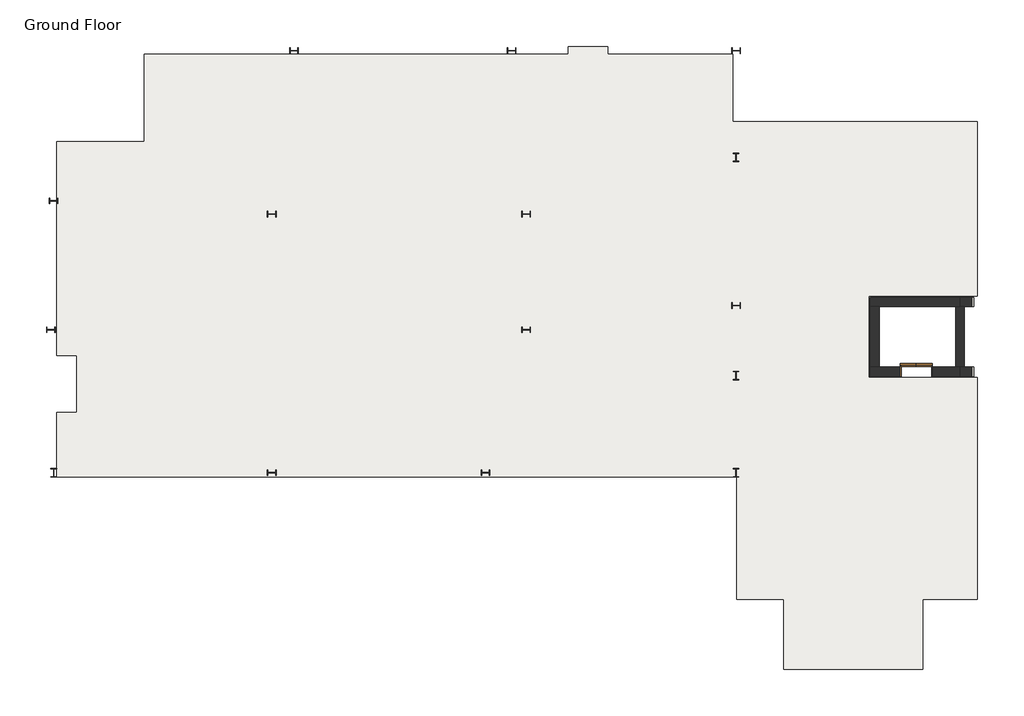
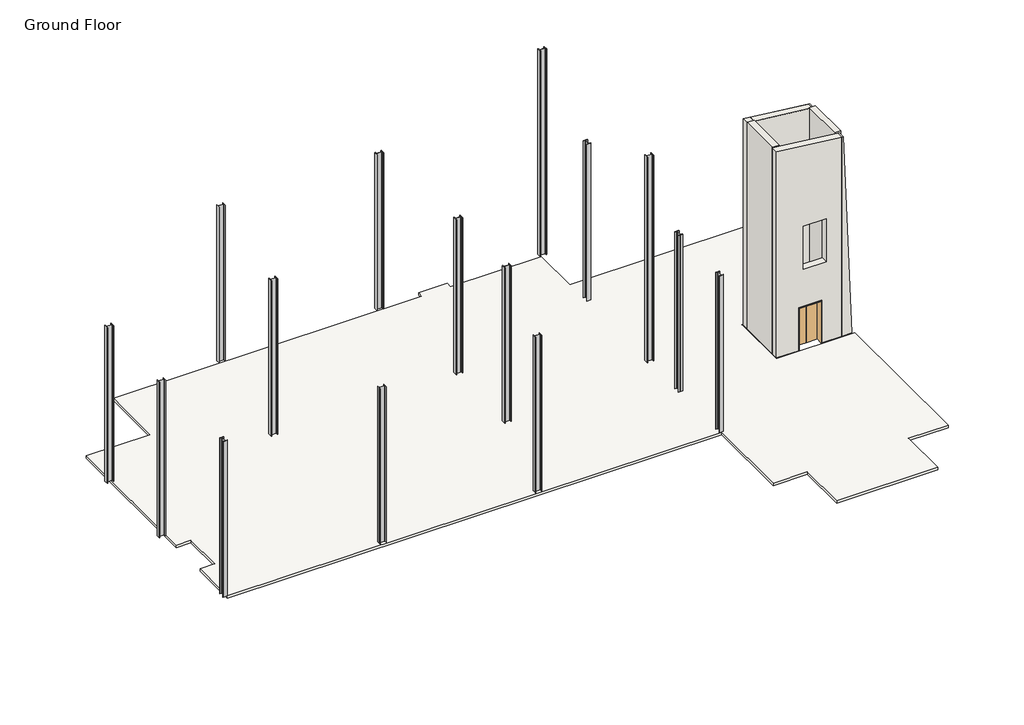
# One storey: 15 columns, 7 walls, 1 door, 1 slab.
"""IFC4 building model written with IfcOpenShell, lengths in millimetres."""

import ifcopenshell
import ifcopenshell.guid

model = None  # the IFC model being written
_history = None  # IfcOwnerHistory: only IFC2X3 demands one
_inside = {}  # id of a spatial element -> (the spatial element, [elements in it])
_under = {}  # id of a project, library or spatial element -> (it, [spatial elements below it])
_declared = {}  # id of a project -> (the project, [libraries it declares])
_typed = {}  # id of a type object -> (the type object, [elements of that type])
_made_of = {}  # id of a material, layer set ... -> (it, [elements and type objects made of it])


def new_model(schema):
    """Start an empty IFC model of exactly this schema.

    Asked for "IFC4X3", IfcOpenShell would pick the latest addendum, in which some entities
    have other attributes; the version numbers below select the first issue.
    IFC2X3 requires an IfcOwnerHistory on every rooted entity: one is made here for all.
    """
    global model, _history
    if schema == "IFC4X3":
        model = ifcopenshell.file(schema_version=(4, 3, 0, 0))
    else:
        model = ifcopenshell.file(schema=schema)
    _inside.clear()
    _under.clear()
    _declared.clear()
    _typed.clear()
    _made_of.clear()
    _history = None
    if model.schema == "IFC2X3":
        org = make("IfcOrganization", Name="unknown")
        user = make(
            "IfcPersonAndOrganization",
            ThePerson=make("IfcPerson", FamilyName="unknown"),
            TheOrganization=org,
        )
        app = make(
            "IfcApplication",
            ApplicationDeveloper=org,
            Version="unknown",
            ApplicationFullName="unknown",
            ApplicationIdentifier="unknown",
        )
        _history = make(
            "IfcOwnerHistory",
            OwningUser=user,
            OwningApplication=app,
            ChangeAction="ADDED",
            CreationDate=0,
        )
    return model


def make(cls, **values):
    """One entity of the class cls with the attributes given. An attribute that is None is left unset."""
    return model.create_entity(
        cls, **{name: value for name, value in values.items() if value is not None}
    )


def rooted(cls, **values):
    """An entity with a GlobalId (a new one), such as an element, a storey or a relation."""
    return make(cls, GlobalId=ifcopenshell.guid.new(), OwnerHistory=_history, **values)


def si_unit(unit_type, name, prefix=None):
    """IfcSIUnit, for example si_unit("LENGTHUNIT", "METRE", prefix="MILLI")."""
    return make("IfcSIUnit", UnitType=unit_type, Prefix=prefix, Name=name)


def assignment(units):
    """IfcUnitAssignment: the units of a project."""
    return None if units is None else make("IfcUnitAssignment", Units=units)


def point(xyz):
    """IfcCartesianPoint."""
    return None if xyz is None else make("IfcCartesianPoint", Coordinates=xyz)


def direction(xyz):
    """IfcDirection."""
    return None if xyz is None else make("IfcDirection", DirectionRatios=xyz)


def frame(location, z_axis=None, x_axis=None):
    """IfcAxis2Placement3D, a coordinate frame: its origin and axes. An axis left out is left unset."""
    return make(
        "IfcAxis2Placement3D",
        Location=point(location),
        Axis=direction(z_axis),
        RefDirection=direction(x_axis),
    )


def frame_2d(location, x_axis=None):
    """IfcAxis2Placement2D, a coordinate frame in the plane: its origin and x axis."""
    return make(
        "IfcAxis2Placement2D", Location=point(location), RefDirection=direction(x_axis)
    )


def origin():
    """The frame at (0, 0, 0) with its axes left unset."""
    return frame((0.0, 0.0, 0.0))


def origin_with_axes():
    """The frame at (0, 0, 0) with the z axis (0, 0, 1) and the x axis (1, 0, 0) written out."""
    return frame((0.0, 0.0, 0.0), z_axis=(0.0, 0.0, 1.0), x_axis=(1.0, 0.0, 0.0))


def place(relative_to, where):
    """IfcLocalPlacement: puts the frame where relative to a parent placement (None: the world)."""
    return make(
        "IfcLocalPlacement", PlacementRelTo=relative_to, RelativePlacement=where
    )


def context(
    kind, dimensions, precision=None, world=None, true_north=None, identifier=None
):
    """IfcGeometricRepresentationContext, for example the 3D "Model" context."""
    return make(
        "IfcGeometricRepresentationContext",
        ContextIdentifier=identifier,
        ContextType=kind,
        CoordinateSpaceDimension=dimensions,
        Precision=precision,
        WorldCoordinateSystem=world,
        TrueNorth=true_north,
    )


def project(units=None, contexts=None):
    """IfcProject with its units and contexts."""
    return rooted(
        "IfcProject",
        Name="project",
        RepresentationContexts=contexts,
        UnitsInContext=assignment(units),
    )


def spatial(cls, under=None, at=None, **own):
    """A site, building, storey or space (cls), placed at a placement, below another one or the project."""
    s = rooted(cls, ObjectPlacement=at, **own)
    if under is not None:
        _under.setdefault(under.id(), (under, []))[1].append(s)
    return s


def polyline(points):
    """IfcPolyline through the points."""
    return make("IfcPolyline", Points=[point(p) for p in points])


def circle_curve(where, radius):
    """IfcCircle in the frame where."""
    return make("IfcCircle", Position=where, Radius=radius)


def trimmed(basis, trim1, trim2, sense, master):
    """IfcTrimmedCurve: the piece of a basis curve between two trims."""
    return make(
        "IfcTrimmedCurve",
        BasisCurve=basis,
        Trim1=trim1,
        Trim2=trim2,
        SenseAgreement=sense,
        MasterRepresentation=master,
    )


def segment(curve, same_sense, transition):
    """IfcCompositeCurveSegment."""
    return make(
        "IfcCompositeCurveSegment",
        Transition=transition,
        SameSense=same_sense,
        ParentCurve=curve,
    )


def composite_curve(segments, self_intersect=None):
    """IfcCompositeCurve: segments joined end to end."""
    return make("IfcCompositeCurve", Segments=segments, SelfIntersect=self_intersect)


def outline(outer, holes=None, kind="AREA"):
    """IfcArbitraryClosedProfileDef: a profile drawn as a closed curve; with holes, ...WithVoids."""
    if holes is None:
        return make("IfcArbitraryClosedProfileDef", ProfileType=kind, OuterCurve=outer)
    return make(
        "IfcArbitraryProfileDefWithVoids",
        ProfileType=kind,
        OuterCurve=outer,
        InnerCurves=holes,
    )


def extrude(swept, where, along, depth):
    """IfcExtrudedAreaSolid: the profile swept, set in the frame where, extruded along a direction by depth."""
    return make(
        "IfcExtrudedAreaSolid",
        SweptArea=swept,
        Position=where,
        ExtrudedDirection=direction(along),
        Depth=depth,
    )


def faces_of(points, faces, orient=None, outer=None):
    """IfcFace entities. A face is a list of loops; a loop is a list of indices into points, from 0.

    orient and outer hold one flag for each loop. By default every Orientation is true, the
    first loop of a face is its IfcFaceOuterBound and the others are IfcFaceBound.
    """
    made = []
    for i, loops in enumerate(faces):
        bounds = []
        for j, loop in enumerate(loops):
            is_outer = j == 0 if outer is None else outer[i][j]
            bounds.append(
                make(
                    "IfcFaceOuterBound" if is_outer else "IfcFaceBound",
                    Bound=make("IfcPolyLoop", Polygon=[points[k] for k in loop]),
                    Orientation=True if orient is None else orient[i][j],
                )
            )
        made.append(make("IfcFace", Bounds=bounds))
    return made


def faceted_brep(points, faces, orient=None, outer=None, voids=None):
    """IfcFacetedBrep: a solid bounded by flat faces; with voids (closed shells), ...WithVoids."""
    shared = [point(p) for p in points]
    hull = make("IfcClosedShell", CfsFaces=faces_of(shared, faces, orient, outer))
    if voids is None:
        return make("IfcFacetedBrep", Outer=hull)
    return make(
        "IfcFacetedBrepWithVoids",
        Outer=hull,
        Voids=[
            make(cls, CfsFaces=faces_of(shared, fs, o, b)) for cls, fs, o, b in voids
        ],
    )


def shape(context_of_items, identifier, shape_type, items):
    """IfcShapeRepresentation: the items that make up one representation, for example the "Body"."""
    return make(
        "IfcShapeRepresentation",
        ContextOfItems=context_of_items,
        RepresentationIdentifier=identifier,
        RepresentationType=shape_type,
        Items=items,
    )


def source(mapping_origin, context_of_items, identifier, shape_type, items):
    """IfcRepresentationMap: a shape defined once, which mapped items show again and again."""
    return make(
        "IfcRepresentationMap",
        MappingOrigin=mapping_origin,
        MappedRepresentation=shape(context_of_items, identifier, shape_type, items),
    )


def transform(
    local_origin,
    x_axis=None,
    y_axis=None,
    z_axis=None,
    scale=None,
    scale2=None,
    scale3=None,
    uniform=True,
):
    """IfcCartesianTransformationOperator3D, or its non-uniform kind. x_axis, y_axis, z_axis: its Axis1, 2, 3."""
    if uniform:
        return make(
            "IfcCartesianTransformationOperator3D",
            Axis1=direction(x_axis),
            Axis2=direction(y_axis),
            LocalOrigin=point(local_origin),
            Scale=scale,
            Axis3=direction(z_axis),
        )
    return make(
        "IfcCartesianTransformationOperator3DnonUniform",
        Axis1=direction(x_axis),
        Axis2=direction(y_axis),
        LocalOrigin=point(local_origin),
        Scale=scale,
        Axis3=direction(z_axis),
        Scale2=scale2,
        Scale3=scale3,
    )


def mapped(mapping_source, mapping_target):
    """IfcMappedItem: shows the shape of a source again, moved by a transform."""
    return make(
        "IfcMappedItem", MappingSource=mapping_source, MappingTarget=mapping_target
    )


def made_of(thing, what):
    """Note that an element or type object is made of a material, layer set ...; save() writes the relation."""
    if what is not None:
        _made_of.setdefault(what.id(), (what, []))[1].append(thing)
    return thing


def element(
    cls,
    number,
    at=None,
    inside=None,
    cuts=None,
    type_object=None,
    material=None,
    context=None,
    identifier="Body",
    shape_type=None,
    held_by="IfcProductDefinitionShape",
    body=None,
    shapes=None,
    **own,
):
    """One element of the class cls, such as IfcWall. Its Tag is "e" and its number.

    at: its placement. inside: the storey or other place that contains it. cuts: it is an
    opening in that element (IfcRelVoidsElement). A single representation is given by context,
    identifier, shape_type and body (its items); several are given by shapes. held_by: the class
    of the entity that holds the representations. save() writes the other relations.
    """
    e = rooted(cls, Tag="e%d" % number, ObjectPlacement=at, **own)
    if body is not None:
        shapes = [shape(context, identifier, shape_type, body)]
    if shapes is not None:
        e.Representation = make(held_by, Representations=shapes)
    if inside is not None:
        _inside.setdefault(inside.id(), (inside, []))[1].append(e)
    if cuts is not None:
        rooted(
            "IfcRelVoidsElement", RelatingBuildingElement=cuts, RelatedOpeningElement=e
        )
    if type_object is not None:
        _typed.setdefault(type_object.id(), (type_object, []))[1].append(e)
    return made_of(e, material)


def aggregate(whole, parts):
    """IfcRelAggregates: a whole, such as a stair, and the parts it consists of."""
    return rooted("IfcRelAggregates", RelatingObject=whole, RelatedObjects=parts)


def save(model, path):
    """Write the relations noted so far, then the file.

    IfcRelAggregates (storeys below a building ...), IfcRelContainedInSpatialStructure (elements
    in a storey), IfcRelDefinesByType, IfcRelAssociatesMaterial and IfcRelDeclares: one each for
    every whole, place, type object, material and project.
    """
    for whole, parts in _under.values():
        aggregate(whole, parts)
    for where, things in _inside.values():
        rooted(
            "IfcRelContainedInSpatialStructure",
            RelatedElements=things,
            RelatingStructure=where,
        )
    for kind, things in _typed.values():
        rooted("IfcRelDefinesByType", RelatedObjects=things, RelatingType=kind)
    for what, things in _made_of.values():
        rooted("IfcRelAssociatesMaterial", RelatedObjects=things, RelatingMaterial=what)
    for by, libraries in _declared.values():
        rooted("IfcRelDeclares", RelatingContext=by, RelatedDefinitions=libraries)
    model.write(path)


def w_wide_flange_column_w12x40_bfea6e2c(model_context):
    return source(origin(), model_context, "Body", "SweptSolid", [
        extrude(outline(composite_curve([segment(polyline([(101.6496094, 151.6558594), (101.6496094, 138.5589844), (25.5984375, 138.5589844)]), True, "CONTINUOUS"), segment(trimmed(circle_curve(frame_2d((25.5984375, 116.7308594)), 21.828125), [point((25.5984375, 138.5589844))], [point((3.7703125, 116.7308594))], True, "CARTESIAN"), True, "CONTINUOUS"), segment(polyline([(3.7703125, 116.7308594), (3.7703125, -116.7308594)]), True, "CONTINUOUS"), segment(trimmed(circle_curve(frame_2d((25.5984375, -116.7308594)), 21.828125), [point((3.7703125, -116.7308594))], [point((25.5984375, -138.5589844))], True, "CARTESIAN"), True, "CONTINUOUS"), segment(polyline([(25.5984375, -138.5589844), (101.6496094, -138.5589844), (101.6496094, -151.6558594), (-101.6496094, -151.6558594), (-101.6496094, -138.5589844), (-25.5984375, -138.5589844)]), True, "CONTINUOUS"), segment(trimmed(circle_curve(frame_2d((-25.5984375, -116.7308594)), 21.828125), [point((-25.5984375, -138.5589844))], [point((-3.7703125, -116.7308594))], True, "CARTESIAN"), True, "CONTINUOUS"), segment(polyline([(-3.7703125, -116.7308594), (-3.7703125, 116.7308594)]), True, "CONTINUOUS"), segment(trimmed(circle_curve(frame_2d((-25.5984375, 116.7308594)), 21.828125), [point((-3.7703125, 116.7308594))], [point((-25.5984375, 138.5589844))], True, "CARTESIAN"), True, "CONTINUOUS"), segment(polyline([(-25.5984375, 138.5589844), (-101.6496094, 138.5589844), (-101.6496094, 151.6558594), (101.6496094, 151.6558594)]), True, "CONTINUOUS")], self_intersect=False)), frame((0.0, 0.0, 30480.0), z_axis=(0.0, 0.0, 1.0), x_axis=(1.0, 0.0, 0.0)), (0.0, 0.0, 1.0), 7924.8),
    ])


def door_aaeb5b8c(model_context):
    return source(origin(), model_context, "Body", "SweptSolid", [
        extrude(outline(polyline([(0.0, 234.95), (0.0, 279.4), (558.8, 279.4), (558.8, 234.95), (0.0, 234.95)])), origin_with_axes(), (0.0, 0.0, 1.0), 2184.4),
        extrude(outline(polyline([(0.0, 234.95), (-558.8, 234.95), (-558.8, 279.4), (0.0, 279.4), (0.0, 234.95)])), origin_with_axes(), (0.0, 0.0, 1.0), 2184.4),
        extrude(outline(polyline([(-533.4, -165.1), (-558.8, -165.1), (-558.8, 177.8), (-533.4, 177.8), (-533.4, -165.1)])), origin_with_axes(), (0.0, 0.0, 1.0), 2184.4),
        extrude(outline(polyline([(558.8, -165.1), (533.4, -165.1), (533.4, 177.8), (558.8, 177.8), (558.8, -165.1)])), origin_with_axes(), (0.0, 0.0, 1.0), 2184.4),
        extrude(outline(polyline([(482.6, 165.1), (482.6, -165.1), (-482.6, -165.1), (-482.6, 165.1), (482.6, 165.1)])), frame((0.0, 0.0, 2133.6), z_axis=(0.0, 0.0, 1.0), x_axis=(1.0, 0.0, 0.0)), (0.0, 0.0, 1.0), 50.8),
        extrude(outline(polyline([(0.0, 177.8), (0.0, 222.25), (558.8, 222.25), (558.8, 177.8), (0.0, 177.8)])), origin_with_axes(), (0.0, 0.0, 1.0), 2184.4),
        extrude(outline(polyline([(0.0, 177.8), (-558.8, 177.8), (-558.8, 222.25), (0.0, 222.25), (0.0, 177.8)])), origin_with_axes(), (0.0, 0.0, 1.0), 2184.4),
    ])


model = new_model("IFC4")

# Units and contexts
model_context = context("Model", 3, world=origin())
ifc_project = project(units=[si_unit("LENGTHUNIT", "METRE", prefix="MILLI")], contexts=[model_context])

# Site, building, storey
site = spatial("IfcSite", under=ifc_project)
building = spatial("IfcBuilding", under=site)
storey = spatial("IfcBuildingStorey", under=building, Name="Ground Floor", Elevation=30480.0)

# Columns
placement = place(None, origin())
element("IfcColumn", 1, ObjectType="W-Wide Flange-Column : W12X40", at=placement, inside=storey, context=model_context, shape_type="SweptSolid", body=[
    extrude(outline(composite_curve([segment(polyline([(13669.3791487, -6791.0746401), (13669.3791487, -6804.1715151), (13593.3279768, -6804.1715151)]), True, "CONTINUOUS"), segment(trimmed(circle_curve(frame_2d((13593.3279768, -6825.9996401)), 21.828125), [point((13593.3279768, -6804.1715151))], [point((13571.4998518, -6825.9996401))], True, "CARTESIAN"), True, "CONTINUOUS"), segment(polyline([(13571.4998518, -6825.9996401), (13571.4998518, -7059.4613589)]), True, "CONTINUOUS"), segment(trimmed(circle_curve(frame_2d((13593.3279768, -7059.4613589)), 21.828125), [point((13571.4998518, -7059.4613589))], [point((13593.3279768, -7081.2894839))], True, "CARTESIAN"), True, "CONTINUOUS"), segment(polyline([(13593.3279768, -7081.2894839), (13669.3791487, -7081.2894839), (13669.3791487, -7094.3863589), (13466.0799299, -7094.3863589), (13466.0799299, -7081.2894839), (13542.1311018, -7081.2894839)]), True, "CONTINUOUS"), segment(trimmed(circle_curve(frame_2d((13542.1311018, -7059.4613589)), 21.828125), [point((13542.1311018, -7081.2894839))], [point((13563.9592268, -7059.4613589))], True, "CARTESIAN"), True, "CONTINUOUS"), segment(polyline([(13563.9592268, -7059.4613589), (13563.9592268, -6825.9996401)]), True, "CONTINUOUS"), segment(trimmed(circle_curve(frame_2d((13542.1311018, -6825.9996401)), 21.828125), [point((13563.9592268, -6825.9996401))], [point((13542.1311018, -6804.1715151))], True, "CARTESIAN"), True, "CONTINUOUS"), segment(polyline([(13542.1311018, -6804.1715151), (13466.0799299, -6804.1715151), (13466.0799299, -6791.0746401), (13669.3791487, -6791.0746401)]), True, "CONTINUOUS")], self_intersect=False)), frame((0.0, 0.0, 30480.0), z_axis=(0.0, 0.0, 1.0), x_axis=(1.0, 0.0, 0.0)), (0.0, 0.0, 1.0), 7988.3),
])
element("IfcColumn", 2, ObjectType="W-Wide Flange-Column : W12X40", at=placement, inside=storey, context=model_context, shape_type="SweptSolid", body=[
    extrude(outline(composite_curve([segment(polyline([(-10575.3444063, -1833.0779639), (-10562.2475313, -1833.0779639), (-10562.2475313, -1909.1291357)]), True, "CONTINUOUS"), segment(trimmed(circle_curve(frame_2d((-10540.4194063, -1909.1291357)), 21.828125), [point((-10562.2475313, -1909.1291357))], [point((-10540.4194063, -1930.9572607))], True, "CARTESIAN"), True, "CONTINUOUS"), segment(polyline([(-10540.4194063, -1930.9572607), (-10306.9576875, -1930.9572607)]), True, "CONTINUOUS"), segment(trimmed(circle_curve(frame_2d((-10306.9576875, -1909.1291357)), 21.828125), [point((-10306.9576875, -1930.9572607))], [point((-10285.1295625, -1909.1291357))], True, "CARTESIAN"), True, "CONTINUOUS"), segment(polyline([(-10285.1295625, -1909.1291357), (-10285.1295625, -1833.0779639), (-10272.0326875, -1833.0779639), (-10272.0326875, -2036.3771826), (-10285.1295625, -2036.3771826), (-10285.1295625, -1960.3260107)]), True, "CONTINUOUS"), segment(trimmed(circle_curve(frame_2d((-10306.9576875, -1960.3260107)), 21.828125), [point((-10285.1295625, -1960.3260107))], [point((-10306.9576875, -1938.4978857))], True, "CARTESIAN"), True, "CONTINUOUS"), segment(polyline([(-10306.9576875, -1938.4978857), (-10540.4194063, -1938.4978857)]), True, "CONTINUOUS"), segment(trimmed(circle_curve(frame_2d((-10540.4194063, -1960.3260107)), 21.828125), [point((-10540.4194063, -1938.4978857))], [point((-10562.2475313, -1960.3260107))], True, "CARTESIAN"), True, "CONTINUOUS"), segment(polyline([(-10562.2475313, -1960.3260107), (-10562.2475313, -2036.3771826), (-10575.3444063, -2036.3771826), (-10575.3444063, -1833.0779639)]), True, "CONTINUOUS")], self_intersect=False)), frame((0.0, 0.0, 30480.0), z_axis=(0.0, 0.0, 1.0), x_axis=(1.0, 0.0, 0.0)), (0.0, 0.0, 1.0), 7924.8),
])
element("IfcColumn", 3, ObjectType="W-Wide Flange-Column : W12X40", at=placement, inside=storey, context=model_context, shape_type="SweptSolid", body=[
    extrude(outline(composite_curve([segment(polyline([(13416.0736799, 7944.8941099), (13429.1705549, 7944.8941099), (13429.1705549, 7868.842938)]), True, "CONTINUOUS"), segment(trimmed(circle_curve(frame_2d((13450.9986799, 7868.842938)), 21.828125), [point((13429.1705549, 7868.842938))], [point((13450.9986799, 7847.014813))], True, "CARTESIAN"), True, "CONTINUOUS"), segment(polyline([(13450.9986799, 7847.014813), (13684.4603987, 7847.014813)]), True, "CONTINUOUS"), segment(trimmed(circle_curve(frame_2d((13684.4603987, 7868.842938)), 21.828125), [point((13684.4603987, 7847.014813))], [point((13706.2885237, 7868.842938))], True, "CARTESIAN"), True, "CONTINUOUS"), segment(polyline([(13706.2885237, 7868.842938), (13706.2885237, 7944.8941099), (13719.3853987, 7944.8941099), (13719.3853987, 7741.5948911), (13706.2885237, 7741.5948911), (13706.2885237, 7817.646063)]), True, "CONTINUOUS"), segment(trimmed(circle_curve(frame_2d((13684.4603987, 7817.646063)), 21.828125), [point((13706.2885237, 7817.646063))], [point((13684.4603987, 7839.474188))], True, "CARTESIAN"), True, "CONTINUOUS"), segment(polyline([(13684.4603987, 7839.474188), (13450.9986799, 7839.474188)]), True, "CONTINUOUS"), segment(trimmed(circle_curve(frame_2d((13450.9986799, 7817.646063)), 21.828125), [point((13450.9986799, 7839.474188))], [point((13429.1705549, 7817.646063))], True, "CARTESIAN"), True, "CONTINUOUS"), segment(polyline([(13429.1705549, 7817.646063), (13429.1705549, 7741.5948911), (13416.0736799, 7741.5948911), (13416.0736799, 7944.8941099)]), True, "CONTINUOUS")], self_intersect=False)), frame((0.0, 0.0, 30480.0), z_axis=(0.0, 0.0, 1.0), x_axis=(1.0, 0.0, 0.0)), (0.0, 0.0, 1.0), 10466.7908493),
])
element("IfcColumn", 4, ObjectType="W-Wide Flange-Column : W12X40", at=placement, inside=storey, context=model_context, shape_type="SweptSolid", body=[
    extrude(outline(composite_curve([segment(polyline([(13466.0799299, 3954.6136411), (13466.0799299, 3967.7105161), (13542.1311018, 3967.7105161)]), True, "CONTINUOUS"), segment(trimmed(circle_curve(frame_2d((13542.1311018, 3989.5386411)), 21.828125), [point((13542.1311018, 3967.7105161))], [point((13563.9592268, 3989.5386411))], True, "CARTESIAN"), True, "CONTINUOUS"), segment(polyline([(13563.9592268, 3989.5386411), (13563.9592268, 4223.0003599)]), True, "CONTINUOUS"), segment(trimmed(circle_curve(frame_2d((13542.1311018, 4223.0003599)), 21.828125), [point((13563.9592268, 4223.0003599))], [point((13542.1311018, 4244.8284849))], True, "CARTESIAN"), True, "CONTINUOUS"), segment(polyline([(13542.1311018, 4244.8284849), (13466.0799299, 4244.8284849), (13466.0799299, 4257.9253599), (13669.3791487, 4257.9253599), (13669.3791487, 4244.8284849), (13593.3279768, 4244.8284849)]), True, "CONTINUOUS"), segment(trimmed(circle_curve(frame_2d((13593.3279768, 4223.0003599)), 21.828125), [point((13593.3279768, 4244.8284849))], [point((13571.4998518, 4223.0003599))], True, "CARTESIAN"), True, "CONTINUOUS"), segment(polyline([(13571.4998518, 4223.0003599), (13571.4998518, 3989.5386411)]), True, "CONTINUOUS"), segment(trimmed(circle_curve(frame_2d((13593.3279768, 3989.5386411)), 21.828125), [point((13571.4998518, 3989.5386411))], [point((13593.3279768, 3967.7105161))], True, "CARTESIAN"), True, "CONTINUOUS"), segment(polyline([(13593.3279768, 3967.7105161), (13669.3791487, 3967.7105161), (13669.3791487, 3954.6136411), (13466.0799299, 3954.6136411)]), True, "CONTINUOUS")], self_intersect=False)), frame((0.0, 0.0, 30480.0), z_axis=(0.0, 0.0, 1.0), x_axis=(1.0, 0.0, 0.0)), (0.0, 0.0, 1.0), 7988.3),
])
element("IfcColumn", 5, ObjectType="W-Wide Flange-Column : W12X40", at=placement, inside=storey, context=model_context, shape_type="SweptSolid", body=[
    extrude(outline(composite_curve([segment(polyline([(13719.3853987, -1186.5051089), (13706.2885237, -1186.5051089), (13706.2885237, -1110.453937)]), True, "CONTINUOUS"), segment(trimmed(circle_curve(frame_2d((13684.4603987, -1110.453937)), 21.828125), [point((13706.2885237, -1110.453937))], [point((13684.4603987, -1088.625812))], True, "CARTESIAN"), True, "CONTINUOUS"), segment(polyline([(13684.4603987, -1088.625812), (13450.9986799, -1088.625812)]), True, "CONTINUOUS"), segment(trimmed(circle_curve(frame_2d((13450.9986799, -1110.453937)), 21.828125), [point((13450.9986799, -1088.625812))], [point((13429.1705549, -1110.453937))], True, "CARTESIAN"), True, "CONTINUOUS"), segment(polyline([(13429.1705549, -1110.453937), (13429.1705549, -1186.5051089), (13416.0736799, -1186.5051089), (13416.0736799, -983.2058901), (13429.1705549, -983.2058901), (13429.1705549, -1059.257062)]), True, "CONTINUOUS"), segment(trimmed(circle_curve(frame_2d((13450.9986799, -1059.257062)), 21.828125), [point((13429.1705549, -1059.257062))], [point((13450.9986799, -1081.085187))], True, "CARTESIAN"), True, "CONTINUOUS"), segment(polyline([(13450.9986799, -1081.085187), (13684.4603987, -1081.085187)]), True, "CONTINUOUS"), segment(trimmed(circle_curve(frame_2d((13684.4603987, -1059.257062)), 21.828125), [point((13684.4603987, -1081.085187))], [point((13706.2885237, -1059.257062))], True, "CARTESIAN"), True, "CONTINUOUS"), segment(polyline([(13706.2885237, -1059.257062), (13706.2885237, -983.2058901), (13719.3853987, -983.2058901), (13719.3853987, -1186.5051089)]), True, "CONTINUOUS")], self_intersect=False)), frame((0.0, 0.0, 30480.0), z_axis=(0.0, 0.0, 1.0), x_axis=(1.0, 0.0, 0.0)), (0.0, 0.0, 1.0), 10466.8036839),
])
element("IfcColumn", 6, ObjectType="W-Wide Flange-Column : W12X40", at=placement, inside=storey, context=model_context, shape_type="SweptSolid", body=[
    extrude(outline(composite_curve([segment(polyline([(13669.3791487, -3387.4746401), (13669.3791487, -3400.5715151), (13593.3279768, -3400.5715151)]), True, "CONTINUOUS"), segment(trimmed(circle_curve(frame_2d((13593.3279768, -3422.3996401)), 21.828125), [point((13593.3279768, -3400.5715151))], [point((13571.4998518, -3422.3996401))], True, "CARTESIAN"), True, "CONTINUOUS"), segment(polyline([(13571.4998518, -3422.3996401), (13571.4998518, -3655.8613589)]), True, "CONTINUOUS"), segment(trimmed(circle_curve(frame_2d((13593.3279768, -3655.8613589)), 21.828125), [point((13571.4998518, -3655.8613589))], [point((13593.3279768, -3677.6894839))], True, "CARTESIAN"), True, "CONTINUOUS"), segment(polyline([(13593.3279768, -3677.6894839), (13669.3791487, -3677.6894839), (13669.3791487, -3690.7863589), (13466.0799299, -3690.7863589), (13466.0799299, -3677.6894839), (13542.1311018, -3677.6894839)]), True, "CONTINUOUS"), segment(trimmed(circle_curve(frame_2d((13542.1311018, -3655.8613589)), 21.828125), [point((13542.1311018, -3677.6894839))], [point((13563.9592268, -3655.8613589))], True, "CARTESIAN"), True, "CONTINUOUS"), segment(polyline([(13563.9592268, -3655.8613589), (13563.9592268, -3422.3996401)]), True, "CONTINUOUS"), segment(trimmed(circle_curve(frame_2d((13542.1311018, -3422.3996401)), 21.828125), [point((13563.9592268, -3422.3996401))], [point((13542.1311018, -3400.5715151))], True, "CARTESIAN"), True, "CONTINUOUS"), segment(polyline([(13542.1311018, -3400.5715151), (13466.0799299, -3400.5715151), (13466.0799299, -3387.4746401), (13669.3791487, -3387.4746401)]), True, "CONTINUOUS")], self_intersect=False)), frame((0.0, 0.0, 30480.0), z_axis=(0.0, 0.0, 1.0), x_axis=(1.0, 0.0, 0.0)), (0.0, 0.0, 1.0), 7988.3),
])
w_wide_flange_column_w12x40_shape = w_wide_flange_column_w12x40_bfea6e2c(model_context)
element("IfcColumn", 7, ObjectType="W-Wide Flange-Column : W12X40", at=placement, inside=storey, context=model_context, shape_type="MappedRepresentation", body=[
    mapped(w_wide_flange_column_w12x40_shape, transform((-10327.3204607, -6942.7304995, 0.0), x_axis=(1.0, 0.0, 0.0), y_axis=(0.0, 1.0, 0.0), z_axis=(0.0, 0.0, 1.0))),
])
element("IfcColumn", 8, ObjectType="W-Wide Flange-Column : W12X40", at=placement, inside=storey, context=model_context, shape_type="MappedRepresentation", body=[
    mapped(w_wide_flange_column_w12x40_shape, transform((-2689.8579607, -6942.7304995, 0.0), x_axis=(0.0, 1.0000000000000002, 0.0), y_axis=(-1.0000000000000002, 0.0, 0.0), z_axis=(0.0, 0.0, 1.0))),
])
element("IfcColumn", 9, ObjectType="W-Wide Flange-Column : W12X40", at=placement, inside=storey, context=model_context, shape_type="MappedRepresentation", body=[
    mapped(w_wide_flange_column_w12x40_shape, transform((4795.2045393, -6942.7304995, 0.0), x_axis=(0.0, 1.0000000000000002, 0.0), y_axis=(-1.0000000000000002, 0.0, 0.0), z_axis=(0.0, 0.0, 1.0))),
])
element("IfcColumn", 10, ObjectType="W-Wide Flange-Column : W12X40", at=placement, inside=storey, context=model_context, shape_type="MappedRepresentation", body=[
    mapped(w_wide_flange_column_w12x40_shape, transform((6216.0170393, -1935.7554995, 0.0), x_axis=(0.0, -1.0000000000000007, 0.0), y_axis=(1.0000000000000007, 0.0, 0.0), z_axis=(0.0, 0.0, 1.0))),
])
element("IfcColumn", 11, ObjectType="W-Wide Flange-Column : W12X40", at=placement, inside=storey, context=model_context, shape_type="MappedRepresentation", body=[
    mapped(w_wide_flange_column_w12x40_shape, transform((-2689.8579607, 2125.0695005, 0.0), x_axis=(0.0, 1.0, 0.0), y_axis=(-1.0, 0.0, 0.0), z_axis=(0.0, 0.0, 1.0))),
])
element("IfcColumn", 12, ObjectType="W-Wide Flange-Column : W12X40", at=placement, inside=storey, context=model_context, shape_type="MappedRepresentation", body=[
    mapped(w_wide_flange_column_w12x40_shape, transform((6216.0170393, 2125.0695005, 0.0), x_axis=(0.0, 1.0000000000000002, 0.0), y_axis=(-1.0000000000000002, 0.0, 0.0), z_axis=(0.0, 0.0, 1.0))),
])
element("IfcColumn", 13, ObjectType="W-Wide Flange-Column : W12X40", at=placement, inside=storey, context=model_context, shape_type="MappedRepresentation", body=[
    mapped(w_wide_flange_column_w12x40_shape, transform((-1910.3954607, 7843.2445005, 0.0), x_axis=(0.0, 1.0000000000000002, 0.0), y_axis=(-1.0000000000000002, 0.0, 0.0), z_axis=(0.0, 0.0, 1.0))),
])
element("IfcColumn", 14, ObjectType="W-Wide Flange-Column : W12X40", at=placement, inside=storey, context=model_context, shape_type="MappedRepresentation", body=[
    mapped(w_wide_flange_column_w12x40_shape, transform((5709.6045393, 7843.2445005, 0.0), x_axis=(0.0, 1.0000000000000002, 0.0), y_axis=(-1.0000000000000002, 0.0, 0.0), z_axis=(0.0, 0.0, 1.0))),
])
element("IfcColumn", 15, ObjectType="W-Wide Flange-Column : W12X40", at=placement, inside=storey, context=model_context, shape_type="MappedRepresentation", body=[
    mapped(w_wide_flange_column_w12x40_shape, transform((-10327.3204607, 2582.2695005, 0.0), x_axis=(0.0, 1.0000000000000002, 0.0), y_axis=(-1.0000000000000002, 0.0, 0.0), z_axis=(0.0, 0.0, 1.0))),
])

# Door
door_shape = door_aaeb5b8c(model_context)
element("IfcDoor", 16, ObjectType="Elevator_Door_CabCenter-Genericrfa : 42\" Opening", at=placement, inside=storey, context=model_context, shape_type="MappedRepresentation", body=[
    mapped(door_shape, transform((19883.5486799, -3399.4304995, 30480.0), x_axis=(1.0, 0.0, 0.0), y_axis=(0.0, 1.0, 0.0), z_axis=(0.0, 0.0, 1.0))),
])

# Slab
element("IfcSlab", 17, ObjectType="5\" Concrete", at=placement, inside=storey, context=model_context, shape_type="SweptSolid", body=[
    extrude(outline(polyline([(7700.3295393, 7725.7695005), (7700.3295393, 7992.4695005), (9071.9295393, 7992.4695005), (9071.9295393, 7725.7695005), (13450.2545393, 7725.7695005), (13450.2545393, 5350.8695005), (22019.578935, 5350.8695005), (22019.578935, -757.8304995), (18219.8486799, -757.8304995), (18219.8486799, -3602.6304995), (22019.578935, -3602.6304995), (22019.578935, -11381.3804995), (20105.0545393, -11381.3804995), (20105.0545393, -13826.1304995), (15240.9545393, -13826.1304995), (15240.9545393, -11381.3804995), (13583.6045393, -11381.3804995), (13583.6045393, -7095.1304995), (-10225.7204607, -7095.1304995), (-10225.7204607, -4821.8304995), (-9524.0454607, -4821.8304995), (-9524.0454607, -2837.4554995), (-10225.7204607, -2837.4554995), (-10225.7204607, 4661.8945005), (-7149.1454607, 4661.8945005), (-7149.1454607, 7725.7695005), (7700.3295393, 7725.7695005)])), frame((0.0, 0.0, 30353.0), z_axis=(0.0, 0.0, 1.0), x_axis=(1.0, 0.0, 0.0)), (0.0, 0.0, 1.0), 127.0),
])

# Walls
element("IfcWall", 18, ObjectType="Elevator Wall - 12\" CMU w furring & Wood Planks", at=placement, inside=storey, context=model_context, shape_type="Brep", body=[
    faceted_brep([(18588.1486799, -3234.3304995, 30480.0), (18588.1486799, -1126.1304995, 30480.0), (18588.1486799, -1126.1304995, 40995.6), (18588.1486799, -3234.3304995, 40995.6), (18257.9486799, -3234.3304995, 30480.0), (18257.9486799, -3234.3304995, 40981.1907931), (18257.9486799, -3234.3304995, 40995.6), (18257.9486799, -1126.1304995, 40995.6), (18257.9486799, -1126.1304995, 40981.1907931), (18257.9486799, -1126.1304995, 30480.0)], [[[0, 1, 2, 3]], [[4, 5, 6, 7, 8, 9]], [[1, 0, 4, 9]], [[3, 2, 7, 6]], [[2, 1, 9, 8, 7]], [[0, 3, 6, 5, 4]]]),
])
element("IfcWall", 19, ObjectType="Elevator Wall - 12\" CMU w furring & Wood Planks", at=placement, inside=storey, context=model_context, shape_type="Brep", body=[
    faceted_brep([(18257.9486799, -1126.1304995, 40981.1907931), (18257.9486799, -1126.1304995, 30480.0), (18588.1486799, -1126.1304995, 30480.0), (21255.1486799, -1126.1304995, 30480.0), (21402.7861799, -1126.1304995, 30480.0), (21402.7861799, -1126.1304995, 40629.44646), (18257.9486799, -795.9304995, 30480.0), (18257.9486799, -795.9304995, 40981.1907931), (21402.7861799, -795.9304995, 40629.44646), (21402.7861799, -795.9304995, 30480.0)], [[[0, 1, 2, 3, 4, 5]], [[6, 7, 8, 9]], [[0, 7, 6, 1]], [[4, 3, 2, 1, 6, 9]], [[5, 4, 9, 8]], [[0, 5, 8, 7]]]),
])
element("IfcWall", 20, ObjectType="Elevator Wall - 12\" CMU w furring & Wood Planks", at=placement, inside=storey, context=model_context, shape_type="Brep", body=[
    faceted_brep([(21889.8617513, -3234.3304995, 30480.0), (21550.4236799, -3234.3304995, 30480.0), (21402.7861799, -3234.3304995, 30480.0), (21402.7861799, -3234.3304995, 40629.44646), (21467.4045193, -3234.3304995, 40622.2190167), (21889.8617513, -3564.5304995, 30480.0), (21467.4045193, -3564.5304995, 40622.2190167), (21402.7861799, -3564.5304995, 40629.44646), (21402.7861799, -3564.5304995, 30480.0)], [[[0, 1, 2, 3, 4]], [[5, 6, 7, 8]], [[2, 1, 0, 5, 8]], [[3, 2, 8, 7]], [[4, 3, 7, 6]], [[0, 4, 6, 5]]]),
])
element("IfcWall", 21, ObjectType="Elevator Wall - 12\" CMU w furring & Wood Planks", at=placement, inside=storey, context=model_context, shape_type="Brep", body=[
    faceted_brep([(21402.7861799, -1126.1304995, 30480.0), (21550.4236799, -1126.1304995, 30480.0), (21889.8617513, -1126.1304995, 30480.0), (21467.4045193, -1126.1304995, 40622.2190167), (21402.7861799, -1126.1304995, 40629.44646), (21402.7861799, -795.9304995, 30480.0), (21402.7861799, -795.9304995, 40629.44646), (21467.4045193, -795.9304995, 40622.2190167), (21889.8617513, -795.9304995, 30480.0)], [[[0, 1, 2, 3, 4]], [[5, 6, 7, 8]], [[2, 1, 0, 5, 8]], [[3, 2, 8, 7]], [[4, 3, 7, 6]], [[0, 4, 6, 5]]]),
])
element("IfcWall", 22, ObjectType="Elevator Wall - 12\" CMU w furring & Wood Planks", at=placement, inside=storey, context=model_context, shape_type="Brep", body=[
    faceted_brep([(18257.9486799, -3234.3304995, 40981.1907931), (21402.7861799, -3234.3304995, 40629.44646), (21402.7861799, -3234.3304995, 30480.0), (21255.1486799, -3234.3304995, 30480.0), (20442.3486799, -3234.3304995, 30480.0), (20442.3486799, -3234.3304995, 32664.4), (19324.7486799, -3234.3304995, 32664.4), (19324.7486799, -3234.3304995, 30480.0), (18588.1486799, -3234.3304995, 30480.0), (18257.9486799, -3234.3304995, 30480.0), (20665.8141096, -3234.3304995, 34544.0), (20665.8141096, -3234.3304995, 36728.4), (19548.2141096, -3234.3304995, 36728.4), (19548.2141096, -3234.3304995, 34544.0), (21402.7861799, -3564.5304995, 40629.44646), (18257.9486799, -3564.5304995, 40981.1907931), (18257.9486799, -3564.5304995, 30480.0), (19324.7486799, -3564.5304995, 30480.0), (19324.7486799, -3564.5304995, 32664.4), (20442.3486799, -3564.5304995, 32664.4), (20442.3486799, -3564.5304995, 30480.0), (21402.7861799, -3564.5304995, 30480.0), (20665.8141096, -3564.5304995, 34544.0), (19548.2141096, -3564.5304995, 34544.0), (19548.2141096, -3564.5304995, 36728.4), (20665.8141096, -3564.5304995, 36728.4)], [[[0, 1, 2, 3, 4, 5, 6, 7, 8, 9], [10, 11, 12, 13]], [[14, 15, 16, 17, 18, 19, 20, 21], [22, 23, 24, 25]], [[0, 9, 16, 15]], [[10, 13, 23, 22]], [[13, 12, 24, 23]], [[12, 11, 25, 24]], [[11, 10, 22, 25]], [[19, 5, 4, 20]], [[5, 19, 18, 6]], [[6, 18, 17, 7]], [[16, 9, 8, 7, 17]], [[2, 21, 20, 4, 3]], [[1, 0, 15, 14]], [[2, 1, 14, 21]]]),
])
element("IfcWall", 23, ObjectType="Elevator Wall - 12\" CMU w furring & Wood Planks", at=placement, inside=storey, context=model_context, shape_type="SweptSolid", body=[
    extrude(outline(polyline([(40944.2585259, 18588.1486799), (30480.0, 18588.1486799), (30480.0, 21889.8617513), (40622.2190167, 21467.4045193), (40944.2585259, 18588.1486799)])), frame((0.0, -1126.1304995, 0.0), z_axis=(0.0, 1.0, 0.0), x_axis=(0.0, 0.0, 1.0)), (0.0, 0.0, 1.0), 330.2),
])
element("IfcWall", 24, ObjectType="Elevator Wall - 12\" CMU", at=placement, inside=storey, context=model_context, shape_type="Brep", body=[
    faceted_brep([(21550.4236799, -3234.3304995, 40690.8), (21550.4236799, -3234.3304995, 30480.0), (21550.4236799, -1126.1304995, 30480.0), (21550.4236799, -1126.1304995, 40690.8), (21255.1486799, -3234.3304995, 30480.0), (21255.1486799, -3234.3304995, 40690.8), (21255.1486799, -1126.1304995, 40690.8), (21255.1486799, -1126.1304995, 30480.0), (21402.7861799, -3234.3304995, 30480.0), (21402.7861799, -1126.1304995, 30480.0)], [[[0, 1, 2, 3]], [[4, 5, 6, 7]], [[2, 1, 8, 4, 7, 9]], [[0, 3, 6, 5]], [[2, 9, 7, 6, 3]], [[0, 5, 4, 8, 1]]]),
])

save(model, "model.ifc")

# Revit data of these elements
# Type "W-Wide Flange-Column : W12X40"
#   Assembly Code = "B10"
#   W = 40
#   bf = 203.299 mm
#   d = 303.312 mm
#   k = 34.925 mm
#   kr = 21.828 mm
#   tf = 13.097 mm
#   tw = 7.541 mm
#   A = 0.00761289 m²
#   Structural Material [instance default] = Steel ASTM A992
# Type "Elevator_Door_CabCenter-Genericrfa : 42\" Opening"
#   Type Mark = "22"
#   Fire Rating = "-"
#   Analytic Construction = "<None>"
#   Thickness = 44.45 mm
#   Rough Width = 965.2 mm
#   Rough Height = 2184.4 mm
#   HalfRoughWidthNeg = -482.6 mm
#   HalfRoughWidth = 482.6 mm
#   Trim Projection = 25.4 mm
#   Trim Width = 76.2 mm
#   Height = 2133.6 mm
#   Width = 1066.8 mm
#   Opening Width = 914.4 mm
#   Frame Jamb Thickness = 25.4 mm
#   Frame Head Thickness = 50.8 mm
#   Door Spacing = 57.15 mm
#   Cab Setback [instance default] = 12.7 mm
#   Cab Depth [instance default] = 1371.6 mm
#   Cab Width [instance default] = 2032 mm
#   Trim [instance default] = no
#   Function = (empty or 0)
#   Wall Closure = (empty or 0)
# Type "5\" Concrete"
#   Assembly Code = "B1010"
#   Function = 0
#   Layers, outside or top first: 127 mm "Concrete, Normal Weight - 4 ksi" (function 1)
# Type "Elevator Wall - 12\" CMU w furring & Wood Planks"
#   Assembly Code = "B2010"
#   Type Mark = "ELEV1"
#   Layers, outside or top first: 15.875 mm "Aluminum 7075" (function 4); 19.05 mm "Aluminum 7075" (function 4); 295.275 mm "Aluminum 7075" (function 1)
# Type "Elevator Wall - 12\" CMU"
#   Assembly Code = "B2010"
#   Type Mark = "ELEV3"
#   Layers, outside or top first: 295.275 mm "Concrete Masonry Units" (function 1)
# Element 1 (IfcColumn, "W-Wide Flange-Column : W12X40")
#   Comments = ""
#   RM User Number = 4
#   RM Unique Id = 792
#   RS Unique Id = 269951
#   Structural Material = Aluminum, Anodized Red
#   Phase Created = New Construction
#   Materials on its faces: "Aluminum, Anodized Red"
# Element 2 (IfcColumn, "W-Wide Flange-Column : W12X40")
#   Comments = ""
#   RM User Number = 11
#   RM Unique Id = 799
#   RS Unique Id = 270567
#   Structural Material = Aluminum, Anodized Red
#   Phase Created = New Construction
#   Materials on its faces: "Aluminum, Anodized Red"
# Element 3 (IfcColumn, "W-Wide Flange-Column : W12X40")
#   Comments = ""
#   RM User Number = 13
#   RM Unique Id = 801
#   RS Unique Id = 270790
#   Structural Material = Aluminum, Anodized Red
#   Phase Created = New Construction
#   Materials on its faces: "Aluminum, Anodized Red"
# Element 4 (IfcColumn, "W-Wide Flange-Column : W12X40")
#   Comments = ""
#   RM User Number = 14
#   RM Unique Id = 802
#   RS Unique Id = 270990
#   Structural Material = Aluminum, Anodized Red
#   Phase Created = New Construction
#   Materials on its faces: "Aluminum, Anodized Red"
# Element 5 (IfcColumn, "W-Wide Flange-Column : W12X40")
#   Comments = ""
#   RM User Number = 15
#   RM Unique Id = 803
#   RS Unique Id = 271156
#   Structural Material = Aluminum, Anodized Red
#   Phase Created = New Construction
#   Materials on its faces: "Aluminum, Anodized Red"
# Element 6 (IfcColumn, "W-Wide Flange-Column : W12X40")
#   Comments = ""
#   RM User Number = 16
#   RM Unique Id = 804
#   RS Unique Id = 271666
#   Structural Material = Aluminum, Anodized Red
#   Phase Created = New Construction
#   Materials on its faces: "Aluminum, Anodized Red"
# Element 7 (IfcColumn, "W-Wide Flange-Column : W12X40")
#   Comments = ""
#   RM User Number = 1
#   RM Unique Id = 789
#   RS Unique Id = 269681
#   Structural Material = Aluminum, Anodized Red
#   Phase Created = New Construction
#   Materials on its faces: "Aluminum, Anodized Red"
# Element 8 (IfcColumn, "W-Wide Flange-Column : W12X40")
#   Comments = ""
#   RM User Number = 2
#   RM Unique Id = 790
#   RS Unique Id = 269697
#   Structural Material = Aluminum, Anodized Red
#   Phase Created = New Construction
#   Materials on its faces: "Aluminum, Anodized Red"
# Element 9 (IfcColumn, "W-Wide Flange-Column : W12X40")
#   Comments = ""
#   RM User Number = 3
#   RM Unique Id = 791
#   RS Unique Id = 269787
#   Structural Material = Aluminum, Anodized Red
#   Phase Created = New Construction
#   Materials on its faces: "Aluminum, Anodized Red"
# Element 10 (IfcColumn, "W-Wide Flange-Column : W12X40")
#   Comments = ""
#   RM User Number = 5
#   RM Unique Id = 793
#   RS Unique Id = 269992
#   Structural Material = Aluminum, Anodized Red
#   Phase Created = New Construction
#   Materials on its faces: "Aluminum, Anodized Red"
# Element 11 (IfcColumn, "W-Wide Flange-Column : W12X40")
#   Comments = ""
#   RM User Number = 6
#   RM Unique Id = 794
#   RS Unique Id = 270272
#   Structural Material = Aluminum, Anodized Red
#   Phase Created = New Construction
#   Materials on its faces: "Aluminum, Anodized Red"
# Element 12 (IfcColumn, "W-Wide Flange-Column : W12X40")
#   Comments = ""
#   RM User Number = 7
#   RM Unique Id = 795
#   RS Unique Id = 270317
#   Structural Material = Aluminum, Anodized Red
#   Phase Created = New Construction
#   Materials on its faces: "Aluminum, Anodized Red"
# Element 13 (IfcColumn, "W-Wide Flange-Column : W12X40")
#   Comments = ""
#   RM User Number = 8
#   RM Unique Id = 796
#   RS Unique Id = 270362
#   Structural Material = Aluminum, Anodized Red
#   Phase Created = New Construction
#   Materials on its faces: "Aluminum, Anodized Red"
# Element 14 (IfcColumn, "W-Wide Flange-Column : W12X40")
#   Comments = ""
#   RM User Number = 9
#   RM Unique Id = 797
#   RS Unique Id = 270435
#   Structural Material = Aluminum, Anodized Red
#   Phase Created = New Construction
#   Materials on its faces: "Aluminum, Anodized Red"
# Element 15 (IfcColumn, "W-Wide Flange-Column : W12X40")
#   Comments = ""
#   RM User Number = 10
#   RM Unique Id = 798
#   RS Unique Id = 270482
#   Structural Material = Aluminum, Anodized Red
#   Phase Created = New Construction
#   Materials on its faces: "Aluminum, Anodized Red"
# Element 16 (IfcDoor, "Elevator_Door_CabCenter-Genericrfa : 42\" Opening")
#   Comments = "Based on KONE EdoSpace MRL 3500"
#   Cab Width = 2032 mm
#   Cab Setback = 12.7 mm
#   Cab Depth = 1681.163 mm
#   Trim = no
#   Phase Created = New Construction
#   Materials on its faces: "Door"
# Element 17 (IfcSlab, "5\" Concrete")
#   Height Offset From Level = 0 mm
#   built-in parameter 1001954 = 1
#   RM User Number = 234
#   RM Unique Id = 1058
#   RS Unique Id = 301493
#   Phase Created = New Construction
#   Materials on its faces: "Concrete, Normal Weight - 4 ksi"
# Element 18 (IfcWall, "Elevator Wall - 12\" CMU w furring & Wood Planks")
#   RMObject_Labels = "REINFORCEMENT=Ściana żelbetowa;CALC_MODEL=powłoka"
#   Top Offset = -304.8 mm
#   Base Offset = 0 mm
#   wall height = 10515.6 mm
#   RMPref.MeshParams.SurfaceParams.Delaunay.H0 = 0.3
#   RMPref.MeshParams.SurfaceParams.Delaunay.H_max = 1000
#   RMPref.MeshParams.SurfaceParams.Delaunay.Q = 1.2
#   RMPref.MeshParams.SurfaceParams.FiniteElems.ConversionCoeff = -0.3
#   RMPref.MeshParams.SurfaceParams.Generation.ElementSize = 0.3048
#   RMPref.MeshParams.Flag = 2
#   RMPref.MeshParams.SurfaceParams.Coons.ForcingRatio = 2
#   RMPref.MeshParams.SurfaceParams.Coons.PanelDivisionType = 2
#   RMPref.MeshParams.SurfaceParams.Delaunay.EmittersDefault = -1
#   RMPref.MeshParams.SurfaceParams.Delaunay.EmittersUser = -1
#   RMPref.MeshParams.SurfaceParams.Delaunay.Type = 1
#   RMPref.MeshParams.SurfaceParams.Delaunay.RegularMesh = -1
#   RMPref.MeshParams.SurfaceParams.FiniteElems.ForcingRatio = 4
#   RMPref.MeshParams.SurfaceParams.FiniteElems.Type = 2
#   RMPref.MeshParams.SurfaceParams.Generation.Division1 = 5
#   RMPref.MeshParams.SurfaceParams.Generation.Type = 3
#   RMPref.MeshParams.SurfaceParams.Method.ForcingRatio = 4
#   RMPref.MeshParams.SurfaceParams.Method.ImplementDegree = 1
#   RMPref.MeshParams.SurfaceParams.Method.Method = 2
#   RM User Number = 254
#   RM Unique Id = 1095
#   RS Unique Id = 387222
#   Phase Created = New Construction
#   Base Constraint = Ground Floor
#   Top Constraint = TOS - ATRIUM ROOF
#   Materials on its faces: "Default Wall", "Aluminum 7075"
# Element 19 (IfcWall, "Elevator Wall - 12\" CMU w furring & Wood Planks")
#   RMObject_Labels = "REINFORCEMENT=Ściana żelbetowa;CALC_MODEL=powłoka"
#   Top Offset = 0 mm
#   Base Offset = 0 mm
#   wall height = 10820.4 mm
#   RMPref.MeshParams.SurfaceParams.Delaunay.H0 = 0.3
#   RMPref.MeshParams.SurfaceParams.Delaunay.H_max = 1000
#   RMPref.MeshParams.SurfaceParams.Delaunay.Q = 1.2
#   RMPref.MeshParams.SurfaceParams.FiniteElems.ConversionCoeff = -0.3
#   RMPref.MeshParams.SurfaceParams.Generation.ElementSize = 0.3048
#   RMPref.MeshParams.Flag = 2
#   RMPref.MeshParams.SurfaceParams.Coons.ForcingRatio = 2
#   RMPref.MeshParams.SurfaceParams.Coons.PanelDivisionType = 2
#   RMPref.MeshParams.SurfaceParams.Delaunay.EmittersDefault = -1
#   RMPref.MeshParams.SurfaceParams.Delaunay.EmittersUser = -1
#   RMPref.MeshParams.SurfaceParams.Delaunay.Type = 1
#   RMPref.MeshParams.SurfaceParams.Delaunay.RegularMesh = -1
#   RMPref.MeshParams.SurfaceParams.FiniteElems.ForcingRatio = 4
#   RMPref.MeshParams.SurfaceParams.FiniteElems.Type = 2
#   RMPref.MeshParams.SurfaceParams.Generation.Division1 = 5
#   RMPref.MeshParams.SurfaceParams.Generation.Type = 3
#   RMPref.MeshParams.SurfaceParams.Method.ForcingRatio = 4
#   RMPref.MeshParams.SurfaceParams.Method.ImplementDegree = 1
#   RMPref.MeshParams.SurfaceParams.Method.Method = 2
#   RM User Number = 255
#   RM Unique Id = 1099
#   RS Unique Id = 387223
#   Phase Created = New Construction
#   Base Constraint = Ground Floor
#   Top Constraint = TOS - ATRIUM ROOF
#   Materials on its faces: "Aluminum 7075", "Default Wall"
# Element 20 (IfcWall, "Elevator Wall - 12\" CMU w furring & Wood Planks")
#   RMObject_Labels = "REINFORCEMENT=Ściana żelbetowa;CALC_MODEL=powłoka"
#   Top Offset = 0 mm
#   Base Offset = 0 mm
#   wall height = 10820.4 mm
#   RMPref.MeshParams.SurfaceParams.Delaunay.H0 = 0.3
#   RMPref.MeshParams.SurfaceParams.Delaunay.H_max = 1000
#   RMPref.MeshParams.SurfaceParams.Delaunay.Q = 1.2
#   RMPref.MeshParams.SurfaceParams.FiniteElems.ConversionCoeff = -0.3
#   RMPref.MeshParams.SurfaceParams.Generation.ElementSize = 0.3048
#   RMPref.MeshParams.Flag = 2
#   RMPref.MeshParams.SurfaceParams.Coons.ForcingRatio = 2
#   RMPref.MeshParams.SurfaceParams.Coons.PanelDivisionType = 2
#   RMPref.MeshParams.SurfaceParams.Delaunay.EmittersDefault = -1
#   RMPref.MeshParams.SurfaceParams.Delaunay.EmittersUser = -1
#   RMPref.MeshParams.SurfaceParams.Delaunay.Type = 1
#   RMPref.MeshParams.SurfaceParams.Delaunay.RegularMesh = -1
#   RMPref.MeshParams.SurfaceParams.FiniteElems.ForcingRatio = 4
#   RMPref.MeshParams.SurfaceParams.FiniteElems.Type = 2
#   RMPref.MeshParams.SurfaceParams.Generation.Division1 = 5
#   RMPref.MeshParams.SurfaceParams.Generation.Type = 3
#   RMPref.MeshParams.SurfaceParams.Method.ForcingRatio = 4
#   RMPref.MeshParams.SurfaceParams.Method.ImplementDegree = 1
#   RMPref.MeshParams.SurfaceParams.Method.Method = 2
#   RM User Number = 256
#   RM Unique Id = 1100
#   RS Unique Id = 387224
#   Phase Created = New Construction
#   Base Constraint = Ground Floor
#   Top Constraint = TOS - ATRIUM ROOF
#   Materials on its faces: "Default Wall", "Aluminum 7075"
# Element 21 (IfcWall, "Elevator Wall - 12\" CMU w furring & Wood Planks")
#   RMObject_Labels = "REINFORCEMENT=Ściana żelbetowa;CALC_MODEL=powłoka"
#   Top Offset = 0 mm
#   Base Offset = 0 mm
#   wall height = 10820.4 mm
#   RMPref.MeshParams.SurfaceParams.Delaunay.H0 = 0.3
#   RMPref.MeshParams.SurfaceParams.Delaunay.H_max = 1000
#   RMPref.MeshParams.SurfaceParams.Delaunay.Q = 1.2
#   RMPref.MeshParams.SurfaceParams.FiniteElems.ConversionCoeff = -0.3
#   RMPref.MeshParams.SurfaceParams.Generation.ElementSize = 0.3048
#   RMPref.MeshParams.Flag = 2
#   RMPref.MeshParams.SurfaceParams.Coons.ForcingRatio = 2
#   RMPref.MeshParams.SurfaceParams.Coons.PanelDivisionType = 2
#   RMPref.MeshParams.SurfaceParams.Delaunay.EmittersDefault = -1
#   RMPref.MeshParams.SurfaceParams.Delaunay.EmittersUser = -1
#   RMPref.MeshParams.SurfaceParams.Delaunay.Type = 1
#   RMPref.MeshParams.SurfaceParams.Delaunay.RegularMesh = -1
#   RMPref.MeshParams.SurfaceParams.FiniteElems.ForcingRatio = 4
#   RMPref.MeshParams.SurfaceParams.FiniteElems.Type = 2
#   RMPref.MeshParams.SurfaceParams.Generation.Division1 = 5
#   RMPref.MeshParams.SurfaceParams.Generation.Type = 3
#   RMPref.MeshParams.SurfaceParams.Method.ForcingRatio = 4
#   RMPref.MeshParams.SurfaceParams.Method.ImplementDegree = 1
#   RMPref.MeshParams.SurfaceParams.Method.Method = 2
#   RM User Number = 263
#   RM Unique Id = 1109
#   RS Unique Id = 403600
#   Phase Created = New Construction
#   Base Constraint = Ground Floor
#   Top Constraint = TOS - ATRIUM ROOF
#   Materials on its faces: "Default Wall", "Aluminum 7075"
# Element 22 (IfcWall, "Elevator Wall - 12\" CMU w furring & Wood Planks")
#   RMObject_Labels = "REINFORCEMENT=Ściana żelbetowa;CALC_MODEL=powłoka"
#   Top Offset = 0 mm
#   Base Offset = 0 mm
#   wall height = 10820.4 mm
#   RMPref.MeshParams.SurfaceParams.Delaunay.H0 = 0.3
#   RMPref.MeshParams.SurfaceParams.Delaunay.H_max = 1000
#   RMPref.MeshParams.SurfaceParams.Delaunay.Q = 1.2
#   RMPref.MeshParams.SurfaceParams.FiniteElems.ConversionCoeff = -0.3
#   RMPref.MeshParams.SurfaceParams.Generation.ElementSize = 0.3048
#   RMPref.MeshParams.Flag = 2
#   RMPref.MeshParams.SurfaceParams.Coons.ForcingRatio = 2
#   RMPref.MeshParams.SurfaceParams.Coons.PanelDivisionType = 2
#   RMPref.MeshParams.SurfaceParams.Delaunay.EmittersDefault = -1
#   RMPref.MeshParams.SurfaceParams.Delaunay.EmittersUser = -1
#   RMPref.MeshParams.SurfaceParams.Delaunay.Type = 1
#   RMPref.MeshParams.SurfaceParams.Delaunay.RegularMesh = -1
#   RMPref.MeshParams.SurfaceParams.FiniteElems.ForcingRatio = 4
#   RMPref.MeshParams.SurfaceParams.FiniteElems.Type = 2
#   RMPref.MeshParams.SurfaceParams.Generation.Division1 = 5
#   RMPref.MeshParams.SurfaceParams.Generation.Type = 3
#   RMPref.MeshParams.SurfaceParams.Method.ForcingRatio = 4
#   RMPref.MeshParams.SurfaceParams.Method.ImplementDegree = 1
#   RMPref.MeshParams.SurfaceParams.Method.Method = 2
#   RM User Number = 264
#   RM Unique Id = 1110
#   RS Unique Id = 403681
#   Phase Created = New Construction
#   Base Constraint = Ground Floor
#   Top Constraint = TOS - ATRIUM ROOF
#   Materials on its faces: "Default Wall", "Aluminum 7075"
# Element 23 (IfcWall, "Elevator Wall - 12\" CMU w furring & Wood Planks")
#   Top Offset = 0 mm
#   Base Offset = 0 mm
#   wall height = 10820.4 mm
#   Phase Created = New Construction
#   Base Constraint = Ground Floor
#   Top Constraint = TOS - ATRIUM ROOF
#   Materials on its faces: "Default Wall", "Aluminum 7075"
# Element 24 (IfcWall, "Elevator Wall - 12\" CMU")
#   RMObject_Labels = "REINFORCEMENT=Ściana żelbetowa;CALC_MODEL=powłoka"
#   Top Offset = -609.6 mm
#   Base Offset = 0 mm
#   wall height = 10210.8 mm
#   RMPref.MeshParams.SurfaceParams.Delaunay.H0 = 0.3
#   RMPref.MeshParams.SurfaceParams.Delaunay.H_max = 1000
#   RMPref.MeshParams.SurfaceParams.Delaunay.Q = 1.2
#   RMPref.MeshParams.SurfaceParams.FiniteElems.ConversionCoeff = -0.3
#   RMPref.MeshParams.SurfaceParams.Generation.ElementSize = 0.3048
#   RMPref.MeshParams.Flag = 2
#   RMPref.MeshParams.SurfaceParams.Coons.ForcingRatio = 2
#   RMPref.MeshParams.SurfaceParams.Coons.PanelDivisionType = 2
#   RMPref.MeshParams.SurfaceParams.Delaunay.EmittersDefault = -1
#   RMPref.MeshParams.SurfaceParams.Delaunay.EmittersUser = -1
#   RMPref.MeshParams.SurfaceParams.Delaunay.Type = 1
#   RMPref.MeshParams.SurfaceParams.Delaunay.RegularMesh = -1
#   RMPref.MeshParams.SurfaceParams.FiniteElems.ForcingRatio = 4
#   RMPref.MeshParams.SurfaceParams.FiniteElems.Type = 2
#   RMPref.MeshParams.SurfaceParams.Generation.Division1 = 5
#   RMPref.MeshParams.SurfaceParams.Generation.Type = 3
#   RMPref.MeshParams.SurfaceParams.Method.ForcingRatio = 4
#   RMPref.MeshParams.SurfaceParams.Method.ImplementDegree = 1
#   RMPref.MeshParams.SurfaceParams.Method.Method = 2
#   RM User Number = 258
#   RM Unique Id = 1101
#   RS Unique Id = 387229
#   Phase Created = New Construction
#   Base Constraint = Ground Floor
#   Top Constraint = TOS - ATRIUM ROOF
#   Materials on its faces: "Concrete Masonry Units"
# Materials
#   "Steel ASTM A992": class "Metal", colour RGB 128 0 0, transparency 0, Description = "Structural steel 50ksi", Cost = 0
#   "Concrete, Normal Weight - 4 ksi": class "Concrete", colour RGB 192 192 192, transparency 0, Description = "Concrete 4 ksi", Cost = 0
#   "Aluminum 7075": class "Metal", colour RGB 120 120 120, transparency 0, Description = "Aluminum, annealed, zinc alloy", Cost = 0
#   "Concrete Masonry Units": class "Masonry", colour RGB 227 227 227, transparency 0, Description = "Concrete masonry units", Cost = 0
#   "Aluminum, Anodized Red": class "Metal", colour RGB 120 120 120, transparency 0, Description = "Anodized aluminum, red", Cost = 0
#   "Door": class "Miscellaneous", colour RGB 192 192 192, transparency 0, Cost = 0
#   "Default Wall": class "Miscellaneous", colour RGB 128 128 128, transparency 0
